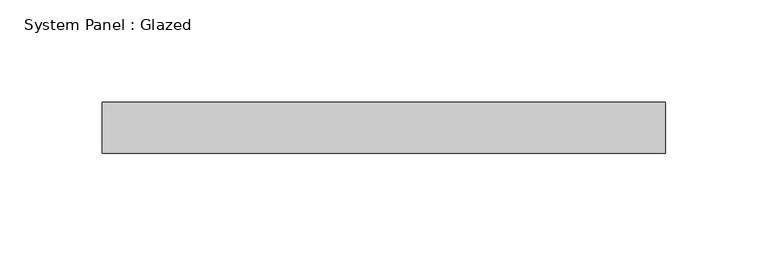
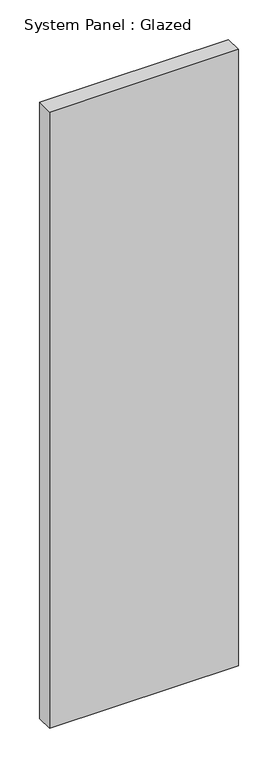
"""IFC4 building model written with IfcOpenShell, lengths in millimetres: plate geometry, System Panel : Glazed."""

from ifc_helpers import new_model, si_unit, origin, origin_with_axes, place, context, project, spatial, polyline, outline, extrude, source, transform, mapped, element, save


def system_panel_glazed_7368e5f6(model_context):
    return source(origin(), model_context, "Body", "SweptSolid", [
        extrude(outline(polyline([(137.8787879, 24.5), (-137.8787879, 24.5), (-137.8787879, 49.5), (137.8787879, 49.5), (137.8787879, 24.5)])), origin_with_axes(), (0.0, 0.0, 1.0), 950.0),
    ])


if __name__ == "__main__":
    model = new_model("IFC4")
    model_context = context("Model", 3, world=origin())
    ifc_project = project(units=[si_unit("LENGTHUNIT", "METRE", prefix="MILLI")], contexts=[model_context])
    site = spatial("IfcSite", under=ifc_project)
    building = spatial("IfcBuilding", under=site)
    placement = place(None, origin())
    system_panel_glazed_shape = system_panel_glazed_7368e5f6(model_context)
    element("IfcPlate", 1, ObjectType="System Panel : Glazed", at=placement, inside=building, context=model_context, shape_type="MappedRepresentation", body=[
        mapped(system_panel_glazed_shape, transform((0.0, 0.0, 0.0), x_axis=(1.0, 0.0, 0.0), y_axis=(0.0, 1.0, 0.0), z_axis=(0.0, 0.0, 1.0))),
    ])
    save(model, "model.ifc")

# Revit data of these elements
# Element 1 (IfcPlate, "System Panel : Glazed")
#   Materials on its faces: "Glass"
# Materials
#   "Glass": class "Glass", colour RGB 218 227 224, transparency 0.85, Description = "Soda Lime Glass", Cost = 0
